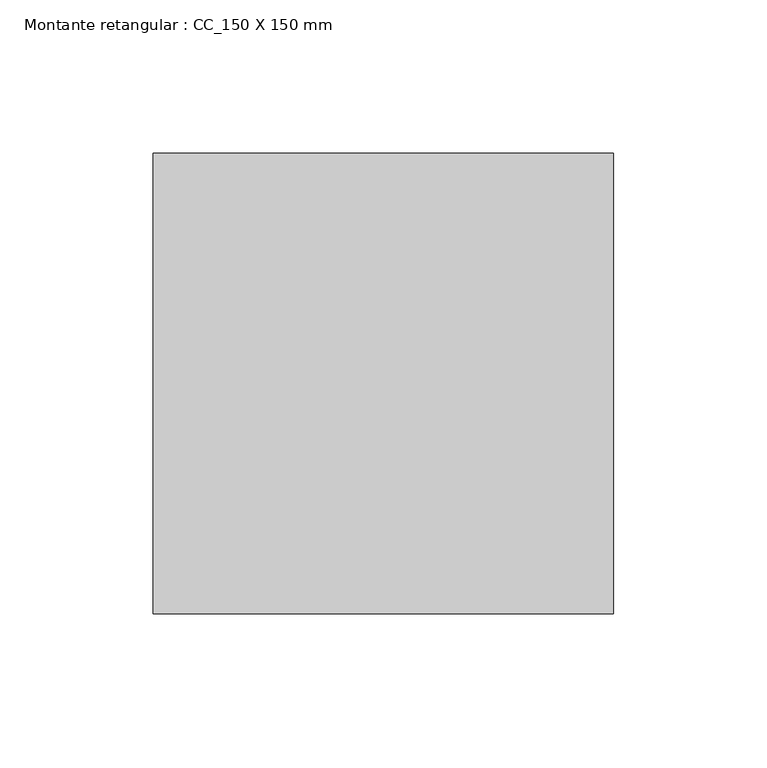
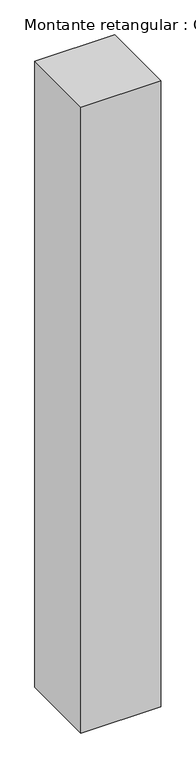
"""IFC4 building model written with IfcOpenShell, lengths in millimetres: member geometry, Montante retangular : CC_150 X 150 mm."""

from ifc_helpers import new_model, si_unit, frame, origin, place, context, project, spatial, polyline, outline, extrude, source, transform, mapped, element, save


def montante_retangular_cc_150_x_150_mm_95775847(model_context):
    return source(origin(), model_context, "Body", "SweptSolid", [
        extrude(outline(polyline([(0.0, 75.0), (0.0, -75.0), (-150.0, -75.0), (-150.0, 75.0), (0.0, 75.0)])), frame((0.0, 0.0, -1243.7499999), z_axis=(0.0, 0.0, 1.0), x_axis=(1.0, 0.0, 0.0)), (0.0, 0.0, 1.0), 1243.7499999),
    ])


if __name__ == "__main__":
    model = new_model("IFC4")
    model_context = context("Model", 3, world=origin())
    ifc_project = project(units=[si_unit("LENGTHUNIT", "METRE", prefix="MILLI")], contexts=[model_context])
    site = spatial("IfcSite", under=ifc_project)
    building = spatial("IfcBuilding", under=site)
    placement = place(None, origin())
    montante_retangular_cc_150_x_150_mm_shape = montante_retangular_cc_150_x_150_mm_95775847(model_context)
    element("IfcMember", 1, ObjectType="Montante retangular : CC_150 X 150 mm", at=placement, inside=building, context=model_context, shape_type="MappedRepresentation", body=[
        mapped(montante_retangular_cc_150_x_150_mm_shape, transform((0.0, 0.0, 0.0), x_axis=(1.0, 0.0, 0.0), y_axis=(0.0, 1.0, 0.0), z_axis=(0.0, 0.0, 1.0))),
    ])
    save(model, "model.ifc")

# Revit data of these elements
# Type "Montante retangular : CC_150 X 150 mm"
#   built-in parameter 1007304 = 0.492126 (stored number, unit not read)
#   built-in parameter 1007301 = 0.246063 (stored number, unit not read)
#   built-in parameter 1007300 = 0.246063 (stored number, unit not read)
# Element 1 (IfcMember, "Montante retangular : CC_150 X 150 mm")
#   Materials on its faces: ".ALUMÍNIO"
# Materials
#   ".ALUMÍNIO": class "CC_METAIS", colour RGB 244 244 244, transparency 0, Description = "Material alumínio", Cost = 0
